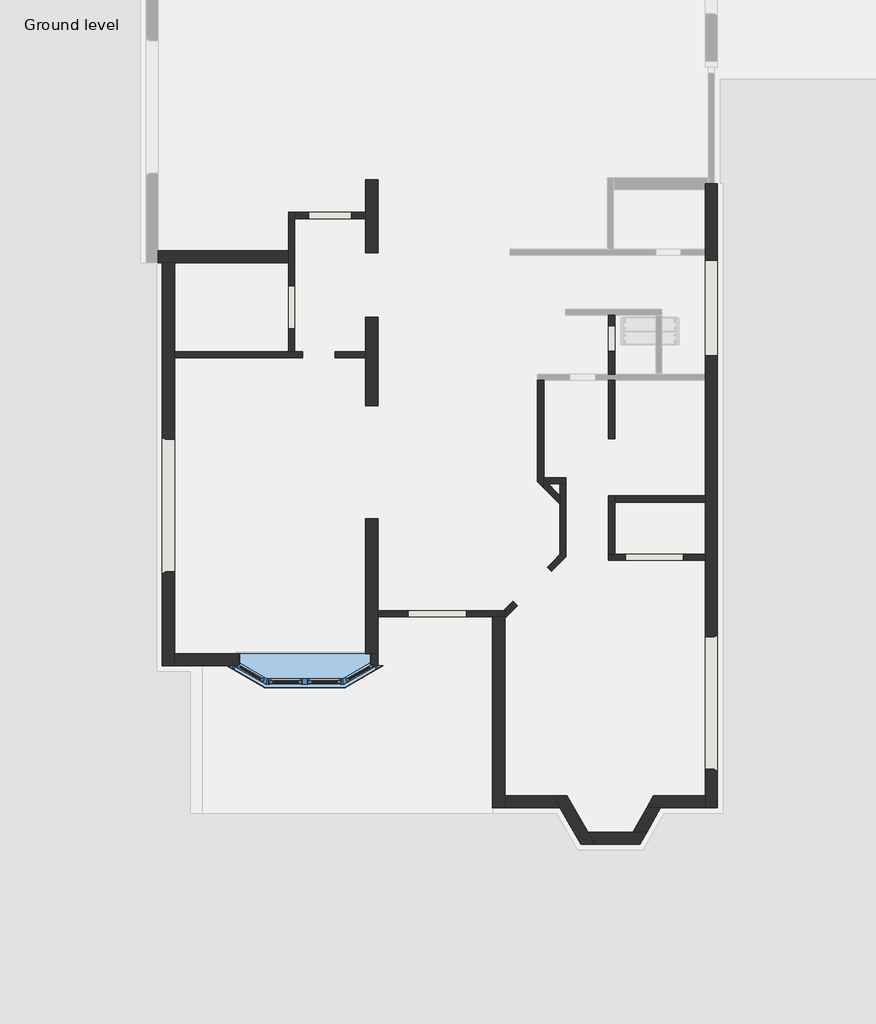
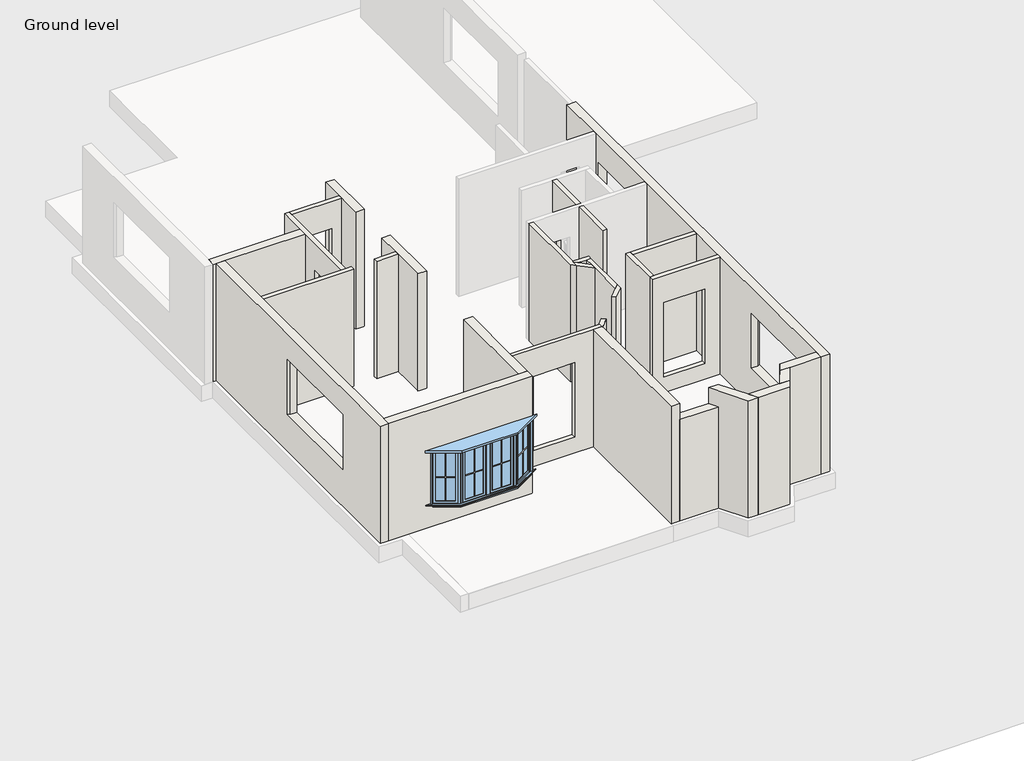
# One storey, part 1 of 2: 28 walls, 1 window.
"""IFC4 building model written with IfcOpenShell, lengths in millimetres."""

import ifcopenshell
import ifcopenshell.guid

model = None  # the IFC model being written
_history = None  # IfcOwnerHistory: only IFC2X3 demands one
_inside = {}  # id of a spatial element -> (the spatial element, [elements in it])
_under = {}  # id of a project, library or spatial element -> (it, [spatial elements below it])
_declared = {}  # id of a project -> (the project, [libraries it declares])
_typed = {}  # id of a type object -> (the type object, [elements of that type])
_made_of = {}  # id of a material, layer set ... -> (it, [elements and type objects made of it])


def new_model(schema):
    """Start an empty IFC model of exactly this schema.

    Asked for "IFC4X3", IfcOpenShell would pick the latest addendum, in which some entities
    have other attributes; the version numbers below select the first issue.
    IFC2X3 requires an IfcOwnerHistory on every rooted entity: one is made here for all.
    """
    global model, _history
    if schema == "IFC4X3":
        model = ifcopenshell.file(schema_version=(4, 3, 0, 0))
    else:
        model = ifcopenshell.file(schema=schema)
    _inside.clear()
    _under.clear()
    _declared.clear()
    _typed.clear()
    _made_of.clear()
    _history = None
    if model.schema == "IFC2X3":
        org = make("IfcOrganization", Name="unknown")
        user = make(
            "IfcPersonAndOrganization",
            ThePerson=make("IfcPerson", FamilyName="unknown"),
            TheOrganization=org,
        )
        app = make(
            "IfcApplication",
            ApplicationDeveloper=org,
            Version="unknown",
            ApplicationFullName="unknown",
            ApplicationIdentifier="unknown",
        )
        _history = make(
            "IfcOwnerHistory",
            OwningUser=user,
            OwningApplication=app,
            ChangeAction="ADDED",
            CreationDate=0,
        )
    return model


def make(cls, **values):
    """One entity of the class cls with the attributes given. An attribute that is None is left unset."""
    return model.create_entity(
        cls, **{name: value for name, value in values.items() if value is not None}
    )


def rooted(cls, **values):
    """An entity with a GlobalId (a new one), such as an element, a storey or a relation."""
    return make(cls, GlobalId=ifcopenshell.guid.new(), OwnerHistory=_history, **values)


def si_unit(unit_type, name, prefix=None):
    """IfcSIUnit, for example si_unit("LENGTHUNIT", "METRE", prefix="MILLI")."""
    return make("IfcSIUnit", UnitType=unit_type, Prefix=prefix, Name=name)


def assignment(units):
    """IfcUnitAssignment: the units of a project."""
    return None if units is None else make("IfcUnitAssignment", Units=units)


def point(xyz):
    """IfcCartesianPoint."""
    return None if xyz is None else make("IfcCartesianPoint", Coordinates=xyz)


def direction(xyz):
    """IfcDirection."""
    return None if xyz is None else make("IfcDirection", DirectionRatios=xyz)


def frame(location, z_axis=None, x_axis=None):
    """IfcAxis2Placement3D, a coordinate frame: its origin and axes. An axis left out is left unset."""
    return make(
        "IfcAxis2Placement3D",
        Location=point(location),
        Axis=direction(z_axis),
        RefDirection=direction(x_axis),
    )


def origin():
    """The frame at (0, 0, 0) with its axes left unset."""
    return frame((0.0, 0.0, 0.0))


def origin_with_axes():
    """The frame at (0, 0, 0) with the z axis (0, 0, 1) and the x axis (1, 0, 0) written out."""
    return frame((0.0, 0.0, 0.0), z_axis=(0.0, 0.0, 1.0), x_axis=(1.0, 0.0, 0.0))


def place(relative_to, where):
    """IfcLocalPlacement: puts the frame where relative to a parent placement (None: the world)."""
    return make(
        "IfcLocalPlacement", PlacementRelTo=relative_to, RelativePlacement=where
    )


def context(
    kind, dimensions, precision=None, world=None, true_north=None, identifier=None
):
    """IfcGeometricRepresentationContext, for example the 3D "Model" context."""
    return make(
        "IfcGeometricRepresentationContext",
        ContextIdentifier=identifier,
        ContextType=kind,
        CoordinateSpaceDimension=dimensions,
        Precision=precision,
        WorldCoordinateSystem=world,
        TrueNorth=true_north,
    )


def project(units=None, contexts=None):
    """IfcProject with its units and contexts."""
    return rooted(
        "IfcProject",
        Name="project",
        RepresentationContexts=contexts,
        UnitsInContext=assignment(units),
    )


def spatial(cls, under=None, at=None, **own):
    """A site, building, storey or space (cls), placed at a placement, below another one or the project."""
    s = rooted(cls, ObjectPlacement=at, **own)
    if under is not None:
        _under.setdefault(under.id(), (under, []))[1].append(s)
    return s


def polyline(points):
    """IfcPolyline through the points."""
    return make("IfcPolyline", Points=[point(p) for p in points])


def outline(outer, holes=None, kind="AREA"):
    """IfcArbitraryClosedProfileDef: a profile drawn as a closed curve; with holes, ...WithVoids."""
    if holes is None:
        return make("IfcArbitraryClosedProfileDef", ProfileType=kind, OuterCurve=outer)
    return make(
        "IfcArbitraryProfileDefWithVoids",
        ProfileType=kind,
        OuterCurve=outer,
        InnerCurves=holes,
    )


def extrude(swept, where, along, depth):
    """IfcExtrudedAreaSolid: the profile swept, set in the frame where, extruded along a direction by depth."""
    return make(
        "IfcExtrudedAreaSolid",
        SweptArea=swept,
        Position=where,
        ExtrudedDirection=direction(along),
        Depth=depth,
    )


def faces_of(points, faces, orient=None, outer=None):
    """IfcFace entities. A face is a list of loops; a loop is a list of indices into points, from 0.

    orient and outer hold one flag for each loop. By default every Orientation is true, the
    first loop of a face is its IfcFaceOuterBound and the others are IfcFaceBound.
    """
    made = []
    for i, loops in enumerate(faces):
        bounds = []
        for j, loop in enumerate(loops):
            is_outer = j == 0 if outer is None else outer[i][j]
            bounds.append(
                make(
                    "IfcFaceOuterBound" if is_outer else "IfcFaceBound",
                    Bound=make("IfcPolyLoop", Polygon=[points[k] for k in loop]),
                    Orientation=True if orient is None else orient[i][j],
                )
            )
        made.append(make("IfcFace", Bounds=bounds))
    return made


def faceted_brep(points, faces, orient=None, outer=None, voids=None):
    """IfcFacetedBrep: a solid bounded by flat faces; with voids (closed shells), ...WithVoids."""
    shared = [point(p) for p in points]
    hull = make("IfcClosedShell", CfsFaces=faces_of(shared, faces, orient, outer))
    if voids is None:
        return make("IfcFacetedBrep", Outer=hull)
    return make(
        "IfcFacetedBrepWithVoids",
        Outer=hull,
        Voids=[
            make(cls, CfsFaces=faces_of(shared, fs, o, b)) for cls, fs, o, b in voids
        ],
    )


def shape(context_of_items, identifier, shape_type, items):
    """IfcShapeRepresentation: the items that make up one representation, for example the "Body"."""
    return make(
        "IfcShapeRepresentation",
        ContextOfItems=context_of_items,
        RepresentationIdentifier=identifier,
        RepresentationType=shape_type,
        Items=items,
    )


def source(mapping_origin, context_of_items, identifier, shape_type, items):
    """IfcRepresentationMap: a shape defined once, which mapped items show again and again."""
    return make(
        "IfcRepresentationMap",
        MappingOrigin=mapping_origin,
        MappedRepresentation=shape(context_of_items, identifier, shape_type, items),
    )


def transform(
    local_origin,
    x_axis=None,
    y_axis=None,
    z_axis=None,
    scale=None,
    scale2=None,
    scale3=None,
    uniform=True,
):
    """IfcCartesianTransformationOperator3D, or its non-uniform kind. x_axis, y_axis, z_axis: its Axis1, 2, 3."""
    if uniform:
        return make(
            "IfcCartesianTransformationOperator3D",
            Axis1=direction(x_axis),
            Axis2=direction(y_axis),
            LocalOrigin=point(local_origin),
            Scale=scale,
            Axis3=direction(z_axis),
        )
    return make(
        "IfcCartesianTransformationOperator3DnonUniform",
        Axis1=direction(x_axis),
        Axis2=direction(y_axis),
        LocalOrigin=point(local_origin),
        Scale=scale,
        Axis3=direction(z_axis),
        Scale2=scale2,
        Scale3=scale3,
    )


def mapped(mapping_source, mapping_target):
    """IfcMappedItem: shows the shape of a source again, moved by a transform."""
    return make(
        "IfcMappedItem", MappingSource=mapping_source, MappingTarget=mapping_target
    )


def made_of(thing, what):
    """Note that an element or type object is made of a material, layer set ...; save() writes the relation."""
    if what is not None:
        _made_of.setdefault(what.id(), (what, []))[1].append(thing)
    return thing


def element(
    cls,
    number,
    at=None,
    inside=None,
    cuts=None,
    type_object=None,
    material=None,
    context=None,
    identifier="Body",
    shape_type=None,
    held_by="IfcProductDefinitionShape",
    body=None,
    shapes=None,
    **own,
):
    """One element of the class cls, such as IfcWall. Its Tag is "e" and its number.

    at: its placement. inside: the storey or other place that contains it. cuts: it is an
    opening in that element (IfcRelVoidsElement). A single representation is given by context,
    identifier, shape_type and body (its items); several are given by shapes. held_by: the class
    of the entity that holds the representations. save() writes the other relations.
    """
    e = rooted(cls, Tag="e%d" % number, ObjectPlacement=at, **own)
    if body is not None:
        shapes = [shape(context, identifier, shape_type, body)]
    if shapes is not None:
        e.Representation = make(held_by, Representations=shapes)
    if inside is not None:
        _inside.setdefault(inside.id(), (inside, []))[1].append(e)
    if cuts is not None:
        rooted(
            "IfcRelVoidsElement", RelatingBuildingElement=cuts, RelatedOpeningElement=e
        )
    if type_object is not None:
        _typed.setdefault(type_object.id(), (type_object, []))[1].append(e)
    return made_of(e, material)


def aggregate(whole, parts):
    """IfcRelAggregates: a whole, such as a stair, and the parts it consists of."""
    return rooted("IfcRelAggregates", RelatingObject=whole, RelatedObjects=parts)


def save(model, path):
    """Write the relations noted so far, then the file.

    IfcRelAggregates (storeys below a building ...), IfcRelContainedInSpatialStructure (elements
    in a storey), IfcRelDefinesByType, IfcRelAssociatesMaterial and IfcRelDeclares: one each for
    every whole, place, type object, material and project.
    """
    for whole, parts in _under.values():
        aggregate(whole, parts)
    for where, things in _inside.values():
        rooted(
            "IfcRelContainedInSpatialStructure",
            RelatedElements=things,
            RelatingStructure=where,
        )
    for kind, things in _typed.values():
        rooted("IfcRelDefinesByType", RelatedObjects=things, RelatingType=kind)
    for what, things in _made_of.values():
        rooted("IfcRelAssociatesMaterial", RelatedObjects=things, RelatingMaterial=what)
    for by, libraries in _declared.values():
        rooted("IfcRelDeclares", RelatingContext=by, RelatedDefinitions=libraries)
    model.write(path)


def m_window_bay_casement_30_degree_angle_2500_x_1500_x_350mm_0714d089(model_context):
    return source(origin(), model_context, "Body", "SolidModel", [
        extrude(outline(polyline([(1224.4331255, 149.925), (1221.2581255, 144.4257387), (835.0107955, 367.4257387), (838.1857955, 372.925), (1224.4331255, 149.925)])), frame((0.0, 0.0, 720.65), z_axis=(0.0, 0.0, 1.0), x_axis=(1.0, 0.0, 0.0)), (0.0, 0.0, 1.0), 1360.3),
        extrude(outline(polyline([(1218.0831255, 138.9264774), (1214.9081255, 133.4272161), (828.6607955, 356.4272161), (831.8357955, 361.9264774), (1218.0831255, 138.9264774)])), frame((0.0, 0.0, 720.65), z_axis=(0.0, 0.0, 1.0), x_axis=(1.0, 0.0, 0.0)), (0.0, 0.0, 1.0), 1360.3),
        extrude(outline(polyline([(1417.45, 57.1500001), (1417.45, -503.15), (-57.15, -503.15), (-57.15, 57.1500001), (1417.45, 57.1500001)]), holes=[polyline([(1360.3, -445.9999999), (1360.3, 0.0), (0.0, 0.0), (0.0, -445.9999999), (1360.3, -445.9999999)])]), frame((1208.5581255, 122.4286934, 720.65), z_axis=(0.49999999999999967, 0.8660254037844388, 0.0), x_axis=(0.0, 0.0, 1.0)), (0.0, 0.0, 1.0), 44.45),
        faceted_brep([(714.9835794, 363.4, 2150.8), (1250.0, 54.5081255, 2150.8), (1284.925, 115.0, 2150.8), (1344.7940905, 115.0, 2150.8), (1344.7940905, 117.0963066, 2150.8), (742.2072174, 465.0, 2150.8), (1258.0514774, 93.8536934, 2138.1), (772.8174436, 374.0036934, 2138.1), (804.5674436, 428.9963066, 2138.1), (1289.8014774, 148.8463066, 2138.1), (1222.5036934, 70.3831255, 2119.05), (770.2652276, 331.4831255, 2119.05), (789.3152276, 364.4786934, 2119.05), (1241.5536934, 103.3786934, 2119.05), (772.8174436, 374.0036934, 663.5), (804.5674436, 428.9963066, 663.5), (770.2652276, 331.4831255, 682.55), (789.3152276, 364.4786934, 682.55), (742.2072174, 465.0, 650.8), (1344.7940905, 117.0963066, 650.8), (1344.7940905, 115.0, 650.8), (1284.925, 115.0, 650.8), (1250.0, 54.5081255, 650.8), (714.9835794, 363.4, 650.8), (1258.0514774, 93.8536934, 663.5), (1289.8014774, 148.8463066, 663.5), (1222.5036934, 70.3831255, 682.55), (1241.5536934, 103.3786934, 682.55)], [[[0, 1, 2, 3, 4, 5]], [[6, 7, 8, 9]], [[10, 11, 12, 13]], [[7, 14, 15, 8]], [[11, 16, 17, 12]], [[18, 19, 20, 21, 22, 23]], [[14, 24, 25, 15]], [[16, 26, 27, 17]], [[22, 21, 2, 1]], [[4, 19, 18, 5], [8, 15, 25, 9]], [[9, 25, 24, 6]], [[6, 24, 14, 7], [12, 17, 27, 13]], [[13, 27, 26, 10]], [[1, 0, 23, 22], [10, 26, 16, 11]], [[5, 18, 23, 0]], [[2, 21, 20, 3]], [[3, 20, 19, 4]]]),
        extrude(outline(polyline([(-1224.4331255, 149.925), (-838.1857955, 372.925), (-835.0107955, 367.4257387), (-1221.2581255, 144.4257387), (-1224.4331255, 149.925)])), frame((0.0, 0.0, 720.65), z_axis=(0.0, 0.0, 1.0), x_axis=(1.0, 0.0, 0.0)), (0.0, 0.0, 1.0), 1360.3),
        extrude(outline(polyline([(-1218.0831255, 138.9264774), (-831.8357955, 361.9264774), (-828.6607955, 356.4272161), (-1214.9081255, 133.4272161), (-1218.0831255, 138.9264774)])), frame((0.0, 0.0, 720.65), z_axis=(0.0, 0.0, 1.0), x_axis=(1.0, 0.0, 0.0)), (0.0, 0.0, 1.0), 1360.3),
        extrude(outline(polyline([(1417.45, -57.1500001), (-57.15, -57.1500001), (-57.15, 503.15), (1417.45, 503.15), (1417.45, -57.1500001)]), holes=[polyline([(1360.3, 445.9999999), (0.0, 445.9999999), (0.0, 0.0), (1360.3, 0.0), (1360.3, 445.9999999)])]), frame((-1208.5581255, 122.4286934, 720.65), z_axis=(-0.49999999999999967, 0.8660254037844388, 0.0), x_axis=(0.0, 0.0, 1.0)), (0.0, 0.0, 1.0), 44.45),
        faceted_brep([(-714.9835794, 363.4, 2150.8), (-742.2072174, 465.0, 2150.8), (-1344.7940905, 117.0963066, 2150.8), (-1344.7940905, 115.0, 2150.8), (-1284.925, 115.0, 2150.8), (-1250.0, 54.5081255, 2150.8), (-1258.0514774, 93.8536934, 2138.1), (-1289.8014774, 148.8463066, 2138.1), (-804.5674436, 428.9963066, 2138.1), (-772.8174436, 374.0036934, 2138.1), (-1222.5036934, 70.3831255, 2119.05), (-1241.5536934, 103.3786934, 2119.05), (-789.3152276, 364.4786934, 2119.05), (-770.2652276, 331.4831255, 2119.05), (-804.5674436, 428.9963066, 663.5), (-772.8174436, 374.0036934, 663.5), (-789.3152276, 364.4786934, 682.55), (-770.2652276, 331.4831255, 682.55), (-742.2072174, 465.0, 650.8), (-714.9835794, 363.4, 650.8), (-1250.0, 54.5081255, 650.8), (-1284.925, 115.0, 650.8), (-1344.7940905, 115.0, 650.8), (-1344.7940905, 117.0963066, 650.8), (-1289.8014774, 148.8463066, 663.5), (-1258.0514774, 93.8536934, 663.5), (-1241.5536934, 103.3786934, 682.55), (-1222.5036934, 70.3831255, 682.55)], [[[0, 1, 2, 3, 4, 5]], [[6, 7, 8, 9]], [[10, 11, 12, 13]], [[9, 8, 14, 15]], [[13, 12, 16, 17]], [[18, 19, 20, 21, 22, 23]], [[15, 14, 24, 25]], [[17, 16, 26, 27]], [[20, 5, 4, 21]], [[2, 1, 18, 23], [8, 7, 24, 14]], [[7, 6, 25, 24]], [[6, 9, 15, 25], [12, 11, 26, 16]], [[11, 10, 27, 26]], [[5, 20, 19, 0], [10, 13, 17, 27]], [[1, 0, 19, 18]], [[4, 3, 22, 21]], [[3, 2, 23, 22]]]),
        faceted_brep([(-755.844462, 515.8, 660.4), (-755.844462, 515.8, 653.0697935), (755.844462, 515.8, 653.0697935), (755.844462, 515.8, 660.4), (-742.232643, 465.0, 663.1486341), (-742.232643, 465.0, 660.4), (742.232643, 465.0, 660.4), (742.232643, 465.0, 663.1486341), (-756.218787, 517.197, 654.4483503), (-756.218787, 517.197, 663.1486341), (756.218787, 517.197, 663.1486341), (756.218787, 517.197, 654.4483503), (759.6217417, 529.897, 652.2089977), (-759.6217417, 529.897, 652.2089977), (759.6217417, 529.897, 643.2668038), (-759.6217417, 529.897, 643.2668038), (-758.5600199, 525.9346, 644.7270038), (-758.5600199, 525.9346, 643.2668038), (758.5600199, 525.9346, 643.2668038), (758.5600199, 525.9346, 644.7270038), (-759.1929694, 528.2968, 650.8662705), (-759.1929694, 528.2968, 644.7270038), (759.1929694, 528.2968, 644.7270038), (759.1929694, 528.2968, 650.8662705), (-1450.0504256, 115.0, 660.4), (-1450.0504256, 115.0, 653.0697935), (1450.0504256, 115.0, 660.4), (1348.4504256, 115.0, 660.4), (-1348.4504256, 115.0, 660.4), (-1348.4504256, 115.0, 663.1486341), (1348.4504256, 115.0, 663.1486341), (1452.8444256, 115.0, 663.1486341), (-1452.8444256, 115.0, 663.1486341), (-1452.8444256, 115.0, 654.4483503), (-1478.2444256, 115.0, 652.2089977), (-1478.2444256, 115.0, 643.2668038), (1478.2444256, 115.0, 643.2668038), (1470.3196257, 115.0, 643.2668038), (-1470.3196257, 115.0, 643.2668038), (-1470.3196257, 115.0, 644.7270038), (1470.3196257, 115.0, 644.7270038), (1475.0440256, 115.0, 644.7270038), (-1475.0440256, 115.0, 644.7270038), (-1475.0440256, 115.0, 650.8662705), (1450.0504256, 115.0, 653.0697935), (1452.8444256, 115.0, 654.4483503), (1478.2444256, 115.0, 652.2089977), (1475.0440256, 115.0, 650.8662705)], [[[0, 1, 2, 3]], [[4, 5, 6, 7]], [[8, 9, 10, 11]], [[8, 11, 12, 13]], [[13, 12, 14, 15]], [[16, 17, 18, 19]], [[20, 21, 22, 23]], [[2, 1, 20, 23]], [[1, 0, 24, 25]], [[0, 3, 26, 27, 6, 5, 28, 24]], [[5, 4, 29, 28]], [[4, 7, 30, 31, 10, 9, 32, 29]], [[9, 8, 33, 32]], [[8, 13, 34, 33]], [[13, 15, 35, 34]], [[15, 14, 36, 37, 18, 17, 38, 35]], [[17, 16, 39, 38]], [[16, 19, 40, 41, 22, 21, 42, 39]], [[21, 20, 43, 42]], [[20, 1, 25, 43]], [[3, 2, 44, 26]], [[7, 6, 27, 30]], [[11, 10, 31, 45]], [[12, 11, 45, 46]], [[14, 12, 46, 36]], [[19, 18, 37, 40]], [[23, 22, 41, 47]], [[2, 23, 47, 44]], [[25, 24, 28, 29, 32, 33, 34, 35, 38, 39, 42, 43]], [[27, 26, 44, 47, 41, 40, 37, 36, 46, 45, 31, 30]]]),
        extrude(outline(polyline([(-1320.9541191, 130.875), (-1348.4504256, 115.0), (-1370.6754256, 153.4948292), (-1343.1791191, 169.3698292), (-1320.9541191, 130.875)])), frame((0.0, 0.0, 663.1486341), z_axis=(0.0, 0.0, 1.0), x_axis=(1.0, 0.0, 0.0)), (0.0, 0.0, 1.0), 1497.2513659),
        extrude(outline(polyline([(1320.9541191, 130.875), (1343.1791191, 169.3698292), (1370.6754256, 153.4948292), (1348.4504256, 115.0), (1320.9541191, 130.875)])), frame((0.0, 0.0, 663.1486341), z_axis=(0.0, 0.0, 1.0), x_axis=(1.0, 0.0, 0.0)), (0.0, 0.0, 1.0), 1497.2513659),
        extrude(outline(polyline([(-714.9835794, 363.4), (714.9835794, 363.4), (1237.3, 61.840474), (1237.3, -115.0), (-1237.3, -115.0), (-1237.3, 61.840474), (-714.9835794, 363.4)])), frame((0.0, 0.0, 2138.1), z_axis=(0.0, 0.0, 1.0), x_axis=(1.0, 0.0, 0.0)), (0.0, 0.0, 1.0), 12.7),
        extrude(outline(polyline([(-1250.0, -115.0), (-1250.0, 54.5081255), (-1237.3, 61.840474), (-1237.3, -115.0), (-1250.0, -115.0)])), frame((0.0, 0.0, 650.8), z_axis=(0.0, 0.0, 1.0), x_axis=(1.0, 0.0, 0.0)), (0.0, 0.0, 1.0), 1500.0),
        extrude(outline(polyline([(1250.0, -115.0), (1237.3, -115.0), (1237.3, 61.840474), (1250.0, 54.5081256), (1250.0, -115.0)])), frame((0.0, 0.0, 650.8), z_axis=(0.0, 0.0, 1.0), x_axis=(1.0, 0.0, 0.0)), (0.0, 0.0, 1.0), 1500.0),
        extrude(outline(polyline([(2138.1, -670.1998305), (663.5, -670.1998305), (663.5, -63.5), (2138.1, -63.5), (2138.1, -670.1998305)]), holes=[polyline([(2080.95, -120.65), (720.65, -120.65), (720.65, -613.0498305), (2080.95, -613.0498305), (2080.95, -120.65)])]), frame((0.0, 401.5, 0.0), z_axis=(0.0, 1.0, 0.0), x_axis=(0.0, 0.0, 1.0)), (0.0, 0.0, 1.0), 44.45),
        extrude(outline(polyline([(2138.1, 63.5), (663.5, 63.5), (663.5, 670.1998305), (2138.1, 670.1998305), (2138.1, 63.5)]), holes=[polyline([(2080.95, 613.0498305), (720.65, 613.0498305), (720.65, 120.65), (2080.95, 120.65), (2080.95, 613.0498305)])]), frame((0.0, 401.5, 0.0), z_axis=(0.0, 1.0, 0.0), x_axis=(0.0, 0.0, 1.0)), (0.0, 0.0, 1.0), 44.45),
        extrude(outline(polyline([(1250.0, -115.0), (-1250.0, -115.0), (-1250.0, 54.5081255), (-1326.2, 186.4903971), (-755.8190363, 515.8), (755.8190363, 515.8), (1326.2, 186.4903971), (1250.0, 54.5081256), (1250.0, -115.0)])), frame((0.0, 0.0, 600.0), z_axis=(0.0, 0.0, 1.0), x_axis=(1.0, 0.0, 0.0)), (0.0, 0.0, 1.0), 50.8),
        faceted_brep([(670.1998305, 401.5, 663.5), (670.1998305, 465.0, 663.5), (63.5, 465.0, 663.5), (63.5, 401.5, 663.5), (651.1498305, 363.4, 682.55), (651.1498305, 401.5, 682.55), (82.55, 401.5, 682.55), (82.55, 363.4, 682.55), (682.8998305, 465.0, 650.8), (682.8998305, 363.4, 650.8), (50.8, 363.4, 650.8), (50.8, 465.0, 650.8), (63.5, 465.0, 2138.1), (63.5, 401.5, 2138.1), (82.55, 401.5, 2119.05), (82.55, 363.4, 2119.05), (50.8, 363.4, 2150.8), (50.8, 465.0, 2150.8), (670.1998305, 465.0, 2138.1), (670.1998305, 401.5, 2138.1), (651.1498305, 401.5, 2119.05), (651.1498305, 363.4, 2119.05), (682.8998305, 363.4, 2150.8), (682.8998305, 465.0, 2150.8)], [[[0, 1, 2, 3]], [[4, 5, 6, 7]], [[8, 9, 10, 11]], [[3, 2, 12, 13]], [[7, 6, 14, 15]], [[11, 10, 16, 17]], [[13, 12, 18, 19]], [[15, 14, 20, 21]], [[17, 16, 22, 23]], [[11, 17, 23, 8], [1, 18, 12, 2]], [[19, 18, 1, 0]], [[3, 13, 19, 0], [5, 20, 14, 6]], [[21, 20, 5, 4]], [[9, 22, 16, 10], [7, 15, 21, 4]], [[23, 22, 9, 8]]]),
        extrude(outline(polyline([(613.0498305, 433.25), (613.0498305, 426.9), (120.65, 426.9), (120.65, 433.25), (613.0498305, 433.25)])), frame((0.0, 0.0, 720.65), z_axis=(0.0, 0.0, 1.0), x_axis=(1.0, 0.0, 0.0)), (0.0, 0.0, 1.0), 1360.3),
        extrude(outline(polyline([(613.0498305, 420.55), (613.0498305, 414.2), (120.65, 414.2), (120.65, 420.55), (613.0498305, 420.55)])), frame((0.0, 0.0, 720.65), z_axis=(0.0, 0.0, 1.0), x_axis=(1.0, 0.0, 0.0)), (0.0, 0.0, 1.0), 1360.3),
        extrude(outline(polyline([(-120.65, 433.25), (-120.65, 426.9), (-613.0498305, 426.9), (-613.0498305, 433.25), (-120.65, 433.25)])), frame((0.0, 0.0, 720.65), z_axis=(0.0, 0.0, 1.0), x_axis=(1.0, 0.0, 0.0)), (0.0, 0.0, 1.0), 1360.3),
        extrude(outline(polyline([(-120.65, 420.55), (-120.65, 414.2), (-613.0498305, 414.2), (-613.0498305, 420.55), (-120.65, 420.55)])), frame((0.0, 0.0, 720.65), z_axis=(0.0, 0.0, 1.0), x_axis=(1.0, 0.0, 0.0)), (0.0, 0.0, 1.0), 1360.3),
        faceted_brep([(-63.5, 401.5, 663.5), (-63.5, 465.0, 663.5), (-670.1998305, 465.0, 663.5), (-670.1998305, 401.5, 663.5), (-82.55, 363.4, 682.55), (-82.55, 401.5, 682.55), (-651.1498305, 401.5, 682.55), (-651.1498305, 363.4, 682.55), (-50.8, 465.0, 650.8), (-50.8, 363.4, 650.8), (-682.8998305, 363.4, 650.8), (-682.8998305, 465.0, 650.8), (-670.1998305, 465.0, 2138.1), (-670.1998305, 401.5, 2138.1), (-651.1498305, 401.5, 2119.05), (-651.1498305, 363.4, 2119.05), (-682.8998305, 363.4, 2150.8), (-682.8998305, 465.0, 2150.8), (-63.5, 465.0, 2138.1), (-63.5, 401.5, 2138.1), (-82.55, 401.5, 2119.05), (-82.55, 363.4, 2119.05), (-50.8, 363.4, 2150.8), (-50.8, 465.0, 2150.8)], [[[0, 1, 2, 3]], [[4, 5, 6, 7]], [[8, 9, 10, 11]], [[3, 2, 12, 13]], [[7, 6, 14, 15]], [[11, 10, 16, 17]], [[13, 12, 18, 19]], [[15, 14, 20, 21]], [[17, 16, 22, 23]], [[11, 17, 23, 8], [1, 18, 12, 2]], [[19, 18, 1, 0]], [[3, 13, 19, 0], [5, 20, 14, 6]], [[21, 20, 5, 4]], [[9, 22, 16, 10], [7, 15, 21, 4]], [[23, 22, 9, 8]]]),
        extrude(outline(polyline([(50.8, 465.0), (50.8, 363.4), (-50.8, 363.4), (-50.8, 465.0), (50.8, 465.0)])), frame((0.0, 0.0, 650.8), z_axis=(0.0, 0.0, 1.0), x_axis=(1.0, 0.0, 0.0)), (0.0, 0.0, 1.0), 1500.0),
        extrude(outline(polyline([(-682.8998305, 465.0), (-682.8998305, 363.4), (-714.9835794, 363.4), (-742.2072173, 465.0), (-682.8998305, 465.0)])), frame((0.0, 0.0, 650.8), z_axis=(0.0, 0.0, 1.0), x_axis=(1.0, 0.0, 0.0)), (0.0, 0.0, 1.0), 1500.0),
        extrude(outline(polyline([(742.2072173, 465.0), (714.9835794, 363.4), (682.8998305, 363.4), (682.8998305, 465.0), (742.2072173, 465.0)])), frame((0.0, 0.0, 650.8), z_axis=(0.0, 0.0, 1.0), x_axis=(1.0, 0.0, 0.0)), (0.0, 0.0, 1.0), 1500.0),
        extrude(outline(polyline([(762.6249458, 541.2), (1500.825, 115.0), (-1500.825, 115.0), (-762.6249458, 541.2), (762.6249458, 541.2)])), frame((0.0, 0.0, 2150.8), z_axis=(0.0, 0.0, 1.0), x_axis=(1.0, 0.0, 0.0)), (0.0, 0.0, 1.0), 50.8),
    ])


model = new_model("IFC4")

# Units and contexts
model_context = context("Model", 3, world=origin())
ifc_project = project(units=[si_unit("LENGTHUNIT", "METRE", prefix="MILLI")], contexts=[model_context])

# Site, building, storey
site = spatial("IfcSite", under=ifc_project)
building = spatial("IfcBuilding", under=site)
storey = spatial("IfcBuildingStorey", under=building, Name="Ground level", Elevation=0.0)

# Walls
placement = place(None, origin())
element("IfcWall", 1, ObjectType="Wall-Fnd_115m 2", at=placement, inside=storey, context=model_context, shape_type="Brep", body=[
    faceted_brep([(-6490.0190924, -3738.4860544, 0.0), (-4065.0190924, -3738.4860544, 0.0), (-4065.0190924, -3738.4860544, 3327.4), (-6490.0190924, -3738.4860544, 3327.4), (-6490.0190924, -3623.4860544, 0.0), (-6490.0190924, -3623.4860544, 3327.4), (-4332.0690924, -3623.4860544, 3327.4), (-4217.0690924, -3623.4860544, 3327.4), (-4065.0190924, -3623.4860544, 3327.4), (-4065.0190924, -3623.4860544, 0.0), (-4217.0690924, -3623.4860544, 0.0), (-4332.0690924, -3623.4860544, 0.0)], [[[0, 1, 2, 3]], [[4, 5, 6, 7, 8, 9, 10, 11]], [[1, 0, 4, 11, 10, 9]], [[2, 1, 9, 8]], [[3, 2, 8, 7, 6, 5]], [[0, 3, 5, 4]]]),
])
element("IfcWall", 2, ObjectType="Wall-Fnd_115m 2", at=placement, inside=storey, context=model_context, shape_type="Brep", body=[
    faceted_brep([(-4217.0690924, -3623.4860544, 0.0), (-4217.0690924, -1109.5860544, 0.0), (-4217.0690924, -994.5860544, 0.0), (-4217.0690924, -994.5860544, 3327.4), (-4217.0690924, -1109.5860544, 3327.4), (-4217.0690924, -3623.4860544, 3327.4), (-4217.0690924, -3190.8110544, 450.0), (-4217.0690924, -3190.8110544, 2560.0), (-4217.0690924, -2380.8110544, 2560.0), (-4217.0690924, -2380.8110544, 450.0), (-4332.0690924, -3623.4860544, 0.0), (-4332.0690924, -3623.4860544, 3327.4), (-4332.0690924, -1948.1360544, 3327.4), (-4332.0690924, -1718.1360544, 3327.4), (-4332.0690924, -994.5860544, 3327.4), (-4332.0690924, -994.5860544, 0.0), (-4332.0690924, -1718.1360544, 0.0), (-4332.0690924, -1948.1360544, 0.0), (-4332.0690924, -3190.8110544, 450.0), (-4332.0690924, -2380.8110544, 450.0), (-4332.0690924, -2380.8110544, 2560.0), (-4332.0690924, -3190.8110544, 2560.0)], [[[0, 1, 2, 3, 4, 5], [6, 7, 8, 9]], [[10, 11, 12, 13, 14, 15, 16, 17], [18, 19, 20, 21]], [[2, 1, 0, 10, 17, 16, 15]], [[5, 4, 3, 14, 13, 12, 11]], [[0, 5, 11, 10]], [[3, 2, 15, 14]], [[7, 6, 18, 21]], [[8, 7, 21, 20]], [[9, 8, 20, 19]], [[6, 9, 19, 18]]]),
])
element("IfcWall", 3, ObjectType="Wall-Fnd_115m 2", at=placement, inside=storey, context=model_context, shape_type="SweptSolid", body=[
    extrude(outline(polyline([(0.0, -4217.0690924), (0.0, -2871.9190924), (3327.4, -2871.9190924), (3327.4, -4217.0690924), (0.0, -4217.0690924)]), holes=[polyline([(450.0, -3949.4940924), (2560.0, -3949.4940924), (2560.0, -3139.4940924), (450.0, -3139.4940924), (450.0, -3949.4940924)])]), frame((0.0, -1109.5860544, 0.0), z_axis=(0.0, 1.0, 0.0), x_axis=(0.0, 0.0, 1.0)), (0.0, 0.0, 1.0), 115.0),
])
element("IfcWall", 4, ObjectType="Wall-Fnd_115m 2", at=placement, inside=storey, context=model_context, shape_type="SweptSolid", body=[
    extrude(outline(polyline([(-3455.4190924, -3623.4860544), (-2871.9190924, -3623.4860544), (-2871.9190924, -3738.4860544), (-3455.4190924, -3738.4860544), (-3455.4190924, -3623.4860544)])), origin_with_axes(), (0.0, 0.0, 1.0), 3327.4),
])
element("IfcWall", 5, ObjectType="Wall-Fnd_115m 2", at=placement, inside=storey, context=model_context, shape_type="Brep", body=[
    faceted_brep([(378.4041712, -4170.2860544, 0.0), (378.4041712, -6089.3362626, 0.0), (378.4041712, -6089.3362626, 3327.4), (378.4041712, -4170.2860544, 3327.4), (493.4041712, -4170.2860544, 0.0), (493.4041712, -4170.2860544, 3327.4), (493.4041712, -6008.0189828, 3327.4), (493.4041712, -6041.7017029, 3327.4), (493.4041712, -6204.3362626, 3327.4), (493.4041712, -6204.3362626, 0.0), (493.4041712, -6041.7017029, 0.0), (493.4041712, -6008.0189828, 0.0)], [[[0, 1, 2, 3]], [[4, 5, 6, 7, 8, 9, 10, 11]], [[1, 0, 4, 11, 10, 9]], [[3, 2, 8, 7, 6, 5]], [[0, 3, 5, 4]], [[2, 1, 9, 8]]]),
])
element("IfcWall", 6, ObjectType="Wall-Fnd_115m 2", at=placement, inside=storey, context=model_context, shape_type="Brep", body=[
    faceted_brep([(493.4041712, -6204.3362626, 0.0), (802.6682399, -6513.6003313, 0.0), (802.6682399, -6513.6003313, 3327.4), (493.4041712, -6204.3362626, 3327.4), (493.4041712, -6041.7017029, 0.0), (493.4041712, -6041.7017029, 3327.4), (574.7214511, -6123.0189828, 3327.4), (802.6682399, -6350.9657716, 3327.4), (802.6682399, -6350.9657716, 0.0), (574.7214511, -6123.0189828, 0.0)], [[[0, 1, 2, 3]], [[4, 5, 6, 7, 8, 9]], [[1, 0, 4, 9, 8]], [[3, 2, 7, 6, 5]], [[0, 3, 5, 4]], [[2, 1, 8, 7]]]),
])
element("IfcWall", 7, ObjectType="Wall-Fnd_115m 2", at=placement, inside=storey, context=model_context, shape_type="Brep", body=[
    faceted_brep([(917.6682399, -7343.6091371, 0.0), (802.6682399, -7458.6091371, 0.0), (562.3354193, -7698.9419578, 0.0), (562.3354193, -7698.9419578, 3327.4), (802.6682399, -7458.6091371, 3327.4), (917.6682399, -7343.6091371, 3327.4), (917.6682399, -7506.2436968, 0.0), (917.6682399, -7506.2436968, 3327.4), (643.6526991, -7780.2592376, 3327.4), (643.6526991, -7780.2592376, 0.0)], [[[0, 1, 2, 3, 4, 5]], [[6, 7, 8, 9]], [[2, 1, 0, 6, 9]], [[3, 2, 9, 8]], [[5, 4, 3, 8, 7]], [[0, 5, 7, 6]]]),
])
element("IfcWall", 8, ObjectType="Wall-Fnd_115m 2", at=placement, inside=storey, context=model_context, shape_type="Brep", body=[
    faceted_brep([(802.6682399, -6123.0189828, 0.0), (802.6682399, -6350.9657716, 0.0), (802.6682399, -6513.6003313, 0.0), (802.6682399, -7458.6091371, 0.0), (802.6682399, -7458.6091371, 3327.4), (802.6682399, -6513.6003313, 3327.4), (802.6682399, -6350.9657716, 3327.4), (802.6682399, -6123.0189828, 3327.4), (917.6682399, -6123.0189828, 0.0), (917.6682399, -6123.0189828, 3327.4), (917.6682399, -7343.6091371, 3327.4), (917.6682399, -7343.6091371, 0.0)], [[[0, 1, 2, 3, 4, 5, 6, 7]], [[8, 9, 10, 11]], [[3, 2, 1, 0, 8, 11]], [[7, 6, 5, 4, 10, 9]], [[4, 3, 11, 10]], [[0, 7, 9, 8]]]),
])
element("IfcWall", 9, ObjectType="Wall-Fnd_115m 2", at=placement, inside=storey, context=model_context, shape_type="Brep", body=[
    faceted_brep([(3547.9309076, -7451.6158868, 0.0), (1835.4010752, -7451.6158868, 0.0), (1720.4010752, -7451.6158868, 0.0), (1720.4010752, -7451.6158868, 3327.4), (1835.4010752, -7451.6158868, 3327.4), (3547.9309076, -7451.6158868, 3327.4), (2035.4010752, -7451.6158868, 2560.0), (2035.4010752, -7451.6158868, 450.0), (3135.4010752, -7451.6158868, 450.0), (3135.4010752, -7451.6158868, 2560.0), (3547.9309076, -7566.6158868, 0.0), (3547.9309076, -7566.6158868, 3327.4), (1720.4010752, -7566.6158868, 3327.4), (1720.4010752, -7566.6158868, 0.0), (2035.4010752, -7566.6158868, 2560.0), (3135.4010752, -7566.6158868, 2560.0), (3135.4010752, -7566.6158868, 450.0), (2035.4010752, -7566.6158868, 450.0)], [[[0, 1, 2, 3, 4, 5], [6, 7, 8, 9]], [[10, 11, 12, 13], [14, 15, 16, 17]], [[2, 1, 0, 10, 13]], [[5, 4, 3, 12, 11]], [[0, 5, 11, 10]], [[3, 2, 13, 12]], [[7, 6, 14, 17]], [[8, 7, 17, 16]], [[9, 8, 16, 15]], [[6, 9, 15, 14]]]),
])
element("IfcWall", 10, ObjectType="Wall-Fnd_115m 2", at=placement, inside=storey, context=model_context, shape_type="Brep", body=[
    faceted_brep([(1835.4010752, -7451.6158868, 0.0), (1835.4010752, -6468.0658868, 0.0), (1835.4010752, -6353.0658868, 0.0), (1835.4010752, -6353.0658868, 3327.4), (1835.4010752, -6468.0658868, 3327.4), (1835.4010752, -7451.6158868, 3327.4), (1720.4010752, -7451.6158868, 0.0), (1720.4010752, -7451.6158868, 3327.4), (1720.4010752, -6353.0658868, 3327.4), (1720.4010752, -6353.0658868, 0.0)], [[[0, 1, 2, 3, 4, 5]], [[6, 7, 8, 9]], [[2, 1, 0, 6, 9]], [[5, 4, 3, 8, 7]], [[0, 5, 7, 6]], [[3, 2, 9, 8]]]),
])
element("IfcWall", 11, ObjectType="Wall-Fnd_115m 2", at=placement, inside=storey, context=model_context, shape_type="SweptSolid", body=[
    extrude(outline(polyline([(3547.9309076, -6468.0658868), (1835.4010752, -6468.0658868), (1835.4010752, -6353.0658868), (3547.9309076, -6353.0658868), (3547.9309076, -6468.0658868)])), origin_with_axes(), (0.0, 0.0, 1.0), 3327.4),
])
element("IfcWall", 12, ObjectType="Wall-Fnd_115m 2", at=placement, inside=storey, context=model_context, shape_type="SweptSolid", body=[
    extrude(outline(polyline([(1835.4010752, -5271.2009706), (1720.4010752, -5271.2009706), (1720.4010752, -4170.2860544), (1835.4010752, -4170.2860544), (1835.4010752, -5271.2009706)])), origin_with_axes(), (0.0, 0.0, 1.0), 3327.4),
    extrude(outline(polyline([(-2938.3860544, 3327.4), (-2938.3860544, 0.0), (-4055.2860544, 0.0), (-4055.2860544, 3327.4), (-2938.3860544, 3327.4)]), holes=[polyline([(-3138.3860544, 450.0), (-3138.3860544, 2560.0), (-3618.3860544, 2560.0), (-3618.3860544, 450.0), (-3138.3860544, 450.0)])]), frame((1720.4010752, 0.0, 0.0), z_axis=(1.0, 0.0, 0.0), x_axis=(0.0, 1.0, 0.0)), (0.0, 0.0, 1.0), 115.0),
])
element("IfcWall", 13, ObjectType="Wall-Fnd_115m 2", at=placement, inside=storey, context=model_context, shape_type="Brep", body=[
    faceted_brep([(574.7214511, -6123.0189828, 0.0), (802.6682399, -6123.0189828, 0.0), (917.6682399, -6123.0189828, 0.0), (917.6682399, -6123.0189828, 3327.4), (802.6682399, -6123.0189828, 3327.4), (574.7214511, -6123.0189828, 3327.4), (493.4041712, -6008.0189828, 0.0), (493.4041712, -6008.0189828, 3327.4), (917.6682399, -6008.0189828, 3327.4), (917.6682399, -6008.0189828, 0.0), (493.4041712, -6041.7017029, 0.0), (493.4041712, -6041.7017029, 3327.4)], [[[0, 1, 2, 3, 4, 5]], [[6, 7, 8, 9]], [[2, 1, 0, 10, 6, 9]], [[5, 4, 3, 8, 7, 11]], [[0, 5, 11, 10]], [[11, 7, 6, 10]], [[3, 2, 9, 8]]]),
])
element("IfcWall", 14, ObjectType="Wall-Fnd_115m 2", at=placement, inside=storey, context=model_context, shape_type="Brep", body=[
    faceted_brep([(-2641.9190924, -8640.6860544, 0.0), (-471.6190924, -8640.6860544, 0.0), (-241.6190924, -8640.6860544, 0.0), (-241.6190924, -8640.6860544, 3327.4), (-471.6190924, -8640.6860544, 3327.4), (-2641.9190924, -8640.6860544, 3327.4), (-971.6190924, -8640.6860544, 2560.0), (-971.6190924, -8640.6860544, 450.0), (-2071.6190924, -8640.6860544, 450.0), (-2071.6190924, -8640.6860544, 2560.0), (-2641.9190924, -8525.6860544, 0.0), (-2641.9190924, -8525.6860544, 3327.4), (-264.4086773, -8525.6860544, 3327.4), (-241.6190924, -8525.6860544, 3327.4), (-241.6190924, -8525.6860544, 0.0), (-264.4086773, -8525.6860544, 0.0), (-971.6190924, -8525.6860544, 2560.0), (-2071.6190924, -8525.6860544, 2560.0), (-2071.6190924, -8525.6860544, 450.0), (-971.6190924, -8525.6860544, 450.0)], [[[0, 1, 2, 3, 4, 5], [6, 7, 8, 9]], [[10, 11, 12, 13, 14, 15], [16, 17, 18, 19]], [[2, 1, 0, 10, 15, 14]], [[5, 4, 3, 13, 12, 11]], [[0, 5, 11, 10]], [[3, 2, 14, 13]], [[7, 6, 16, 19]], [[8, 7, 19, 18]], [[9, 8, 18, 17]], [[6, 9, 17, 16]]]),
])
element("IfcWall", 15, ObjectType="Wall-Fnd_115m 2", at=placement, inside=storey, context=model_context, shape_type="Brep", body=[
    faceted_brep([(-241.6190924, -8665.5310291, 0.0), (-2.9257416, -8426.8376783, 0.0), (-2.9257416, -8426.8376783, 3327.4), (-241.6190924, -8665.5310291, 3327.4), (-264.4086773, -8525.6860544, 0.0), (-264.4086773, -8525.6860544, 3327.4), (-84.2430214, -8345.5203985, 3327.4), (-84.2430214, -8345.5203985, 0.0), (-241.6190924, -8640.6860544, 0.0), (-241.6190924, -8525.6860544, 0.0), (-241.6190924, -8525.6860544, 3327.4), (-241.6190924, -8640.6860544, 3327.4)], [[[0, 1, 2, 3]], [[4, 5, 6, 7]], [[1, 0, 8, 9, 4, 7]], [[2, 1, 7, 6]], [[3, 2, 6, 5, 10, 11]], [[0, 3, 11, 10, 9, 8]], [[10, 5, 4, 9]]]),
])
element("IfcWall", 16, ObjectType="Wall-Fnd_230mm 2", at=placement, inside=storey, context=model_context, shape_type="Brep", body=[
    faceted_brep([(-6794.8190924, -1948.1360544, 0.0), (-6720.0190924, -1948.1360544, 0.0), (-6490.0190924, -1948.1360544, 0.0), (-4332.0690924, -1948.1360544, 0.0), (-4332.0690924, -1948.1360544, 3327.4), (-6490.0190924, -1948.1360544, 3327.4), (-6720.0190924, -1948.1360544, 3327.4), (-6794.8190924, -1948.1360544, 3327.4), (-6794.8190924, -1718.1360544, 0.0), (-6794.8190924, -1718.1360544, 3327.4), (-4332.0690924, -1718.1360544, 3327.4), (-4332.0690924, -1718.1360544, 0.0)], [[[0, 1, 2, 3, 4, 5, 6, 7]], [[8, 9, 10, 11]], [[3, 2, 1, 0, 8, 11]], [[7, 6, 5, 4, 10, 9]], [[0, 7, 9, 8]], [[4, 3, 11, 10]]]),
])
element("IfcWall", 17, ObjectType="Wall-Fnd_230mm 2", at=placement, inside=storey, context=model_context, shape_type="Brep", body=[
    faceted_brep([(-6720.0190924, -1948.1360544, 0.0), (-6720.0190924, -9563.1360544, 0.0), (-6720.0190924, -9563.1360544, 3327.4), (-6720.0190924, -1948.1360544, 3327.4), (-6720.0190924, -5250.8860544, 2600.8), (-6720.0190924, -7820.7360544, 2600.8), (-6720.0190924, -7820.7360544, 1050.0), (-6720.0190924, -5250.8860544, 1050.0), (-6490.0190924, -1948.1360544, 0.0), (-6490.0190924, -1948.1360544, 3327.4), (-6490.0190924, -3623.4860544, 3327.4), (-6490.0190924, -3738.4860544, 3327.4), (-6490.0190924, -9333.1360544, 3327.4), (-6490.0190924, -9563.1360544, 3327.4), (-6490.0190924, -9563.1360544, 0.0), (-6490.0190924, -9333.1360544, 0.0), (-6490.0190924, -3738.4860544, 0.0), (-6490.0190924, -3623.4860544, 0.0), (-6490.0190924, -7785.8110544, 2600.8), (-6490.0190924, -5285.8110544, 2600.8), (-6490.0190924, -5285.8110544, 1050.0), (-6490.0190924, -7785.8110544, 1050.0), (-6659.527218, -7785.8110544, 2600.8), (-6659.527218, -5285.8110544, 2600.8), (-6659.527218, -7785.8110544, 1050.0), (-6659.527218, -5285.8110544, 1050.0)], [[[0, 1, 2, 3], [4, 5, 6, 7]], [[8, 9, 10, 11, 12, 13, 14, 15, 16, 17], [18, 19, 20, 21]], [[1, 0, 8, 17, 16, 15, 14]], [[3, 2, 13, 12, 11, 10, 9]], [[0, 3, 9, 8]], [[2, 1, 14, 13]], [[22, 5, 4, 23, 19, 18]], [[24, 21, 20, 25, 7, 6]], [[22, 18, 21, 24]], [[19, 23, 25, 20]], [[23, 4, 7, 25]], [[5, 22, 24, 6]]]),
])
element("IfcWall", 18, ObjectType="Wall-Fnd_230mm 2", at=placement, inside=storey, context=model_context, shape_type="Brep", body=[
    faceted_brep([(-6490.0190924, -9563.1360544, 0.0), (-2641.9190924, -9563.1360544, 0.0), (-2641.9190924, -9563.1360544, 3327.4), (-6490.0190924, -9563.1360544, 3327.4), (-5306.8440924, -9563.1360544, 2150.8), (-2736.9940924, -9563.1360544, 2150.8), (-2736.9940924, -9563.1360544, 600.0), (-5306.8440924, -9563.1360544, 600.0), (-6490.0190924, -9333.1360544, 0.0), (-6490.0190924, -9333.1360544, 3327.4), (-2871.9190924, -9333.1360544, 3327.4), (-2641.9190924, -9333.1360544, 3327.4), (-2641.9190924, -9333.1360544, 0.0), (-2871.9190924, -9333.1360544, 0.0), (-2771.9190924, -9333.1360544, 2150.8), (-5271.9190924, -9333.1360544, 2150.8), (-5271.9190924, -9333.1360544, 600.0), (-2771.9190924, -9333.1360544, 600.0), (-2771.9190924, -9502.6441799, 2150.8), (-5271.9190924, -9502.6441799, 2150.8), (-2771.9190924, -9502.6441799, 600.0), (-5271.9190924, -9502.6441799, 600.0)], [[[0, 1, 2, 3], [4, 5, 6, 7]], [[8, 9, 10, 11, 12, 13], [14, 15, 16, 17]], [[1, 0, 8, 13, 12]], [[3, 2, 11, 10, 9]], [[0, 3, 9, 8]], [[2, 1, 12, 11]], [[18, 5, 4, 19, 15, 14]], [[20, 17, 16, 21, 7, 6]], [[18, 14, 17, 20]], [[15, 19, 21, 16]], [[19, 4, 7, 21]], [[5, 18, 20, 6]]]),
])
element("IfcWall", 19, ObjectType="Wall-Fnd_230mm 2", at=placement, inside=storey, context=model_context, shape_type="Brep", body=[
    faceted_brep([(666.7431322, -12017.8360544, 0.0), (799.5336941, -12247.8360544, 0.0), (1199.5336941, -12940.6563774, 0.0), (1199.5336941, -12940.6563774, 3327.4), (666.7431322, -12017.8360544, 3327.4), (666.7431322, -12017.8360544, 2877.4), (932.324256, -12017.8360544, 0.0), (932.324256, -12017.8360544, 3327.4), (1332.324256, -12710.6563774, 3327.4), (1465.1148179, -12940.6563774, 3327.4), (1465.1148179, -12940.6563774, 0.0), (1332.324256, -12710.6563774, 0.0)], [[[0, 1, 2, 3, 4, 5]], [[6, 7, 8, 9, 10, 11]], [[2, 1, 0, 6, 11, 10]], [[4, 3, 9, 8, 7]], [[3, 2, 10, 9]], [[0, 5, 4, 7, 6]]]),
])
element("IfcWall", 20, ObjectType="Wall-Fnd_230mm 2", at=placement, inside=storey, context=model_context, shape_type="Brep", body=[
    faceted_brep([(3547.9309076, -450.5860544, 3327.4), (3547.9309076, -450.5860544, 1294.5462794), (3547.9309076, -450.5860544, 0.0), (3547.9309076, -565.5860544, 0.0), (3547.9309076, -1693.0860544, 0.0), (3547.9309076, -1808.0860544, 0.0), (3547.9309076, -4055.2860544, 0.0), (3547.9309076, -4170.2860544, 0.0), (3547.9309076, -6353.0658868, 0.0), (3547.9309076, -6468.0658868, 0.0), (3547.9309076, -7451.6158868, 0.0), (3547.9309076, -7566.6158868, 0.0), (3547.9309076, -12017.8360544, 0.0), (3547.9309076, -12247.8360544, 0.0), (3547.9309076, -12247.8360544, 3327.4), (3547.9309076, -12017.8360544, 3327.4), (3547.9309076, -7566.6158868, 3327.4), (3547.9309076, -7451.6158868, 3327.4), (3547.9309076, -6468.0658868, 3327.4), (3547.9309076, -6353.0658868, 3327.4), (3547.9309076, -4170.2860544, 3327.4), (3547.9309076, -4055.2860544, 3327.4), (3547.9309076, -1808.0860544, 3327.4), (3547.9309076, -1693.0860544, 3327.4), (3547.9309076, -3705.2860544, 2560.0), (3547.9309076, -3705.2860544, 450.0), (3547.9309076, -1895.2860544, 450.0), (3547.9309076, -1895.2860544, 2560.0), (3547.9309076, -9017.8360544, 2600.8), (3547.9309076, -11517.8360544, 2600.8), (3547.9309076, -11517.8360544, 1050.0), (3547.9309076, -9017.8360544, 1050.0), (3777.9309076, -450.5860544, 0.0), (3777.9309076, -450.5860544, 3327.4), (3777.9309076, -12247.8360544, 3327.4), (3777.9309076, -12247.8360544, 0.0), (3777.9309076, -3705.2860544, 2560.0), (3777.9309076, -1895.2860544, 2560.0), (3777.9309076, -1895.2860544, 450.0), (3777.9309076, -3705.2860544, 450.0), (3777.9309076, -11552.7610544, 2600.8), (3777.9309076, -8982.9110544, 2600.8), (3777.9309076, -8982.9110544, 1050.0), (3777.9309076, -11552.7610544, 1050.0), (3605.4309076, -450.5860544, 0.0), (3720.4309076, -450.5860544, 0.0), (3720.4309076, -450.5860544, 3327.4), (3605.4309076, -450.5860544, 3327.4), (3717.4390331, -9017.8360544, 2600.8), (3717.4390331, -11517.8360544, 2600.8), (3717.4390331, -9017.8360544, 1050.0), (3717.4390331, -11517.8360544, 1050.0)], [[[0, 1, 2, 3, 4, 5, 6, 7, 8, 9, 10, 11, 12, 13, 14, 15, 16, 17, 18, 19, 20, 21, 22, 23], [24, 25, 26, 27], [28, 29, 30, 31]], [[32, 33, 34, 35], [36, 37, 38, 39], [40, 41, 42, 43]], [[13, 12, 11, 10, 9, 8, 7, 6, 5, 4, 3, 2, 44, 45, 32, 35]], [[0, 23, 22, 21, 20, 19, 18, 17, 16, 15, 14, 34, 33, 46, 47]], [[14, 13, 35, 34]], [[0, 47, 46, 33, 32, 45, 44, 2, 1]], [[25, 24, 36, 39]], [[26, 25, 39, 38]], [[27, 26, 38, 37]], [[24, 27, 37, 36]], [[48, 41, 40, 49, 29, 28]], [[50, 31, 30, 51, 43, 42]], [[48, 28, 31, 50]], [[29, 49, 51, 30]], [[49, 40, 43, 51]], [[41, 48, 50, 42]]]),
])
element("IfcWall", 21, ObjectType="Wall-Fnd_230mm 2", at=placement, inside=storey, context=model_context, shape_type="Brep", body=[
    faceted_brep([(3547.9309076, -12017.8360544, 0.0), (2569.9753794, -12017.8360544, 0.0), (2569.9753794, -12017.8360544, 3327.4), (3547.9309076, -12017.8360544, 3327.4), (3547.9309076, -12247.8360544, 0.0), (3547.9309076, -12247.8360544, 3327.4), (2704.4903008, -12247.8360544, 3327.4), (2440.6003794, -12247.8360544, 3327.4), (2440.6003794, -12247.8360544, 0.0), (2704.4903008, -12247.8360544, 0.0)], [[[0, 1, 2, 3]], [[4, 5, 6, 7, 8, 9]], [[1, 0, 4, 9, 8]], [[3, 2, 7, 6, 5]], [[0, 3, 5, 4]], [[2, 1, 8, 7]]]),
])
element("IfcWall", 22, ObjectType="Wall-Fnd_230mm 2", at=placement, inside=storey, context=model_context, shape_type="Brep", body=[
    faceted_brep([(1465.1148179, -12940.6563774, 0.0), (2314.7788691, -12940.6563774, 0.0), (2314.7788691, -12940.6563774, 3327.4), (1465.1148179, -12940.6563774, 3327.4), (1332.324256, -12710.6563774, 0.0), (1332.324256, -12710.6563774, 3327.4), (2180.2639477, -12710.6563774, 3327.4), (2444.1538691, -12710.6563774, 3327.4), (2444.1538691, -12710.6563774, 0.0), (2180.2639477, -12710.6563774, 0.0)], [[[0, 1, 2, 3]], [[4, 5, 6, 7, 8, 9]], [[1, 0, 4, 9, 8]], [[3, 2, 7, 6, 5]], [[0, 3, 5, 4]], [[2, 1, 8, 7]]]),
])
element("IfcWall", 23, ObjectType="Wall-Fnd_230mm 2", at=placement, inside=storey, context=model_context, shape_type="SweptSolid", body=[
    extrude(outline(polyline([(2704.4903008, -12247.8360544), (2444.1538691, -12710.6563774), (2180.2639477, -12710.6563774), (2440.6003794, -12247.8360544), (2704.4903008, -12247.8360544)])), origin_with_axes(), (0.0, 0.0, 1.0), 3327.4),
])
element("IfcWall", 24, ObjectType="Wall-Fnd_230mm 2", at=placement, inside=storey, context=model_context, shape_type="Brep", body=[
    faceted_brep([(-2641.9190924, -9333.1360544, 0.0), (-2641.9190924, -8640.6860544, 0.0), (-2641.9190924, -8525.6860544, 0.0), (-2641.9190924, -6786.1360544, 0.0), (-2641.9190924, -6786.1360544, 3327.4), (-2641.9190924, -8525.6860544, 3327.4), (-2641.9190924, -8640.6860544, 3327.4), (-2641.9190924, -9333.1360544, 3327.4), (-2871.9190924, -9333.1360544, 0.0), (-2871.9190924, -9333.1360544, 3327.4), (-2871.9190924, -6786.1360544, 3327.4), (-2871.9190924, -6786.1360544, 0.0)], [[[0, 1, 2, 3, 4, 5, 6, 7]], [[8, 9, 10, 11]], [[3, 2, 1, 0, 8, 11]], [[4, 3, 11, 10]], [[7, 6, 5, 4, 10, 9]], [[0, 7, 9, 8]]]),
])
element("IfcWall", 25, ObjectType="Wall-Fnd_230mm 2", at=placement, inside=storey, context=model_context, shape_type="Brep", body=[
    faceted_brep([(-2641.9190924, -4652.5360544, 0.0), (-2641.9190924, -2976.1360544, 0.0), (-2641.9190924, -2976.1360544, 3327.4), (-2641.9190924, -4652.5360544, 3327.4), (-2871.9190924, -4652.5360544, 0.0), (-2871.9190924, -4652.5360544, 3327.4), (-2871.9190924, -3738.4860544, 3327.4), (-2871.9190924, -3623.4860544, 3327.4), (-2871.9190924, -2976.1360544, 3327.4), (-2871.9190924, -2976.1360544, 0.0), (-2871.9190924, -3623.4860544, 0.0), (-2871.9190924, -3738.4860544, 0.0)], [[[0, 1, 2, 3]], [[4, 5, 6, 7, 8, 9, 10, 11]], [[1, 0, 4, 11, 10, 9]], [[2, 1, 9, 8]], [[3, 2, 8, 7, 6, 5]], [[0, 3, 5, 4]]]),
])
element("IfcWall", 26, ObjectType="Wall-Fnd_230mm 2", at=placement, inside=storey, context=model_context, shape_type="Brep", body=[
    faceted_brep([(-241.6190924, -12247.8360544, 0.0), (-241.6190924, -12017.8360544, 0.0), (-241.6190924, -8665.5310291, 0.0), (-241.6190924, -8640.6860544, 0.0), (-241.6190924, -8640.6860544, 3327.4), (-241.6190924, -8665.5310291, 3327.4), (-241.6190924, -12247.8360544, 3327.4), (-241.6190924, -12247.8360544, 2877.4), (-471.6190924, -12247.8360544, 0.0), (-471.6190924, -12247.8360544, 3327.4), (-471.6190924, -8640.6860544, 3327.4), (-471.6190924, -8640.6860544, 0.0)], [[[0, 1, 2, 3, 4, 5, 6, 7]], [[8, 9, 10, 11]], [[3, 2, 1, 0, 8, 11]], [[6, 5, 4, 10, 9]], [[4, 3, 11, 10]], [[0, 7, 6, 9, 8]]]),
])
element("IfcWall", 27, ObjectType="Wall-Fnd_230mm 2", at=placement, inside=storey, context=model_context, shape_type="Brep", body=[
    faceted_brep([(-2871.9190924, -372.6360544, 0.0), (-2871.9190924, -994.5860544, 0.0), (-2871.9190924, -1109.5860544, 0.0), (-2871.9190924, -1756.9360544, 0.0), (-2871.9190924, -1756.9360544, 3327.4), (-2871.9190924, -1109.5860544, 3327.4), (-2871.9190924, -994.5860544, 3327.4), (-2871.9190924, -372.6360544, 3327.4), (-2641.9190924, -372.6360544, 0.0), (-2641.9190924, -372.6360544, 3327.4), (-2641.9190924, -1756.9360544, 3327.4), (-2641.9190924, -1756.9360544, 0.0)], [[[0, 1, 2, 3, 4, 5, 6, 7]], [[8, 9, 10, 11]], [[3, 2, 1, 0, 8, 11]], [[4, 3, 11, 10]], [[7, 6, 5, 4, 10, 9]], [[0, 7, 9, 8]]]),
])
element("IfcWall", 28, ObjectType="Wall-Fnd_230mm 2", at=placement, inside=storey, context=model_context, shape_type="SweptSolid", body=[
    extrude(outline(polyline([(799.5336941, -12247.8360544), (-241.6190924, -12247.8360544), (-241.6190924, -12017.8360544), (666.7431322, -12017.8360544), (799.5336941, -12247.8360544)])), origin_with_axes(), (0.0, 0.0, 1.0), 2877.4),
])

# Window
m_window_bay_casement_30_degree_angle_2500_x_1500_x_350mm_shape = m_window_bay_casement_30_degree_angle_2500_x_1500_x_350mm_0714d089(model_context)
element("IfcWindow", 29, ObjectType="M_Window-Bay-Casement-30_Degree_Angle : 2500 x 1500 x 350mm", at=placement, inside=storey, context=model_context, shape_type="MappedRepresentation", body=[
    mapped(m_window_bay_casement_30_degree_angle_2500_x_1500_x_350mm_shape, transform((-4021.9190924, -9448.1360544, 0.0), x_axis=(-1.0, 0.0, 0.0), y_axis=(0.0, -1.0, 0.0), z_axis=(0.0, 0.0, 1.0))),
])

save(model, "model.ifc")

# Revit data of these elements
# Project information
#   Project Issue Date = "Issue Date"
#   Project Status = "Project Status"
#   Client Name = "Owner"
#   Project Address = "Enter address here"
#   Project Name = "Project Name"
#   Project Number = "Project Number"
# Type "Wall-Fnd_115m 2"
#   Keynote = "F10"
#   Layers, outside or top first: 115 mm "Concrete Masonry Units" (function 1)
# Type "Wall-Fnd_230mm 2"
#   Keynote = "F10"
#   Layers, outside or top first: 230 mm "Concrete Masonry Units" (function 1)
# Type "M_Window-Bay-Casement-30_Degree_Angle : 2500 x 1500 x 350mm"
#   Type Mark = "50"
#   Fire Rating = "0.5h"
#   Assembly Code = "B2020100"
#   Analytic Construction = "Double glazing - domestic"
#   Width of Middle Sash = 1365.8 mm
#   Width = 2500 mm
#   Visual Light Transmittance = 0.81
#   Thermal Resistance (R) = 0.319569 (m²·K)/W
#   Solar Heat Gain Coefficient = 0.76
#   Rough Width = 2515 mm
#   Rough Height = 1515 mm
#   Length 2 = 1484.465 mm
#   Length 1 = 516.3 mm
#   Wall Thickness [instance default] = 150 mm
#   Trim Width = 2618.666 mm
#   Trim Height = 1500 mm
#   Height 1 = 1550.8 mm
#   Height = 1500 mm
#   Heat Transfer Coefficient (U) = 3.12929 W/(m²·K)
#   Depth = 350 mm
#   Default Sill Height = 600 mm
#   Angle = 30.00°
#   Muntin Visibility = yes
#   Interior Trim Visibility [instance default] = yes
#   Exterior Trim Visibility [instance default] = yes
#   Muntin Pattern = M_Muntin Pattern_2x2 : M_Muntin Pattern_2x2
#   Interior Trim Material = Wood - Stained
#   Exterior Trim Material = Clad - White
#   Exterior Trim = element 343235
#   Interior Trim = M_Trim-Window-Interior-Flat : Picture Frame
#   Interior Frame Material = Wood - Stained
#   Glass Panel Material = Glass
#   Exterior Frame Material = Clad - White
#   Wall Closure = (empty or 0)
# Elements 1, 2, 3, 4, 5, 6, 7, 8, 9, 10, 11, 12, 13, 14, 15 (IfcWall, "Wall-Fnd_115m 2")
#   Top Offset = 0 mm
#   Base Offset = 0 mm
#   Unconnected Height = 3327.4 mm
#   wall height = 3327.4 mm
#   Phase Created = New Construction
#   Base Constraint = Ground level
#   Materials on its faces: "Concrete Masonry Units"
# Elements 16, 17, 18, 19, 20, 21, 22, 23, 24, 25, 26, 27 (IfcWall, "Wall-Fnd_230mm 2")
#   Top Offset = 0 mm
#   Base Offset = 0 mm
#   Unconnected Height = 3327.4 mm
#   wall height = 3327.4 mm
#   Phase Created = New Construction
#   Base Constraint = Ground level
#   Materials on its faces: "Concrete Masonry Units"
# Element 28 (IfcWall, "Wall-Fnd_230mm 2")
#   Top Offset = 0 mm
#   Base Offset = 0 mm
#   Unconnected Height = 2877.4 mm
#   wall height = 2877.4 mm
#   Phase Created = New Construction
#   Base Constraint = Ground level
#   Materials on its faces: "Concrete Masonry Units"
# Element 29 (IfcWindow, "M_Window-Bay-Casement-30_Degree_Angle : 2500 x 1500 x 350mm")
#   Mark = "19"
#   Interior Trim Visibility = yes
#   Exterior Trim Visibility = yes
#   Phase Created = New Construction
#   Materials on its faces: "Clad - White", "Wood - Stained", "Glass"
# Materials
#   "Concrete Masonry Units": class "Masonry", colour RGB 181 181 181, transparency 0, Description = "Concrete masonry units", Cost = 0
#   "Wood - Stained": class "Wood", colour RGB 227 170 128, transparency 0, Cost = 0
#   "Clad - White": class "Wood", colour RGB 242 242 238, transparency 0, Cost = 0
#   "Glass": class "Glass", colour RGB 0 128 192, transparency 0.9, Description = "Soda Lime Glass", Cost = 0
# Room at (0, 7730.579) mm, phase "New Construction", upper level "Ground level", upper offset 4000 mm, lower offset 0 mm
#   Number = "1"
#   Name = "Room"
# Room at (-5346.219, -2701.787) mm, phase "New Construction", upper level "Ground level", upper offset 4000 mm, lower offset 0 mm
#   Number = "room 2"
#   Name = "Room"
# Room at (0, 3710.442) mm, phase "New Construction", upper level "Ground level", upper offset 4000 mm, lower offset 0 mm
#   Number = "10"
#   Name = "Room"
# Room at (-4370.719, 2184.354) mm, phase "New Construction", upper level "Ground level", upper offset 4000 mm, lower offset 0 mm
#   Number = "11"
#   Name = "Room"
# Room at (-1012, -6499.299) mm, phase "New Construction", upper level "Ground level", upper offset 4000 mm, lower offset 0 mm
#   Number = "12"
#   Name = "Room"
# Room at (2720.416, -6959.841) mm, phase "New Construction", upper level "Ground level", upper offset 4000 mm, lower offset 0 mm
#   Number = "29"
#   Name = "Room"
# Room at (2225.116, -3496.836) mm, phase "New Construction", upper level "Ground level", upper offset 4000 mm, lower offset 0 mm
#   Number = "30"
#   Name = "Room"
# Room at (2710.431, -1100.586) mm, phase "New Construction", upper level "Ground level", upper offset 4000 mm, lower offset 0 mm
#   Number = "31"
#   Name = "Room"
